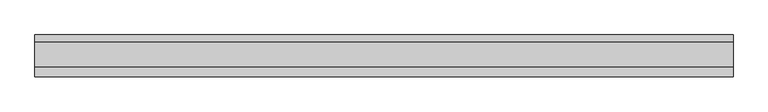
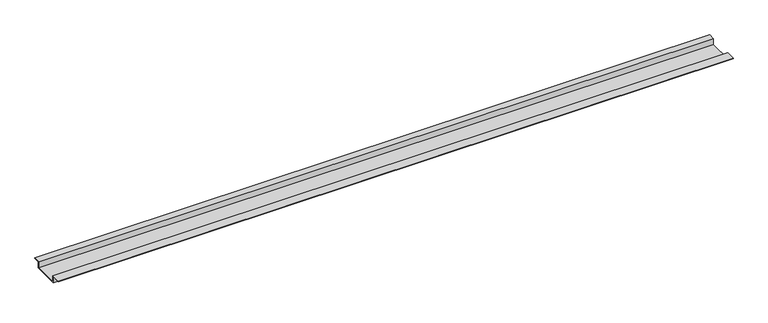
"""IFC4 building model written with IfcOpenShell, lengths in millimetres: proxy geometry, Soffit004 5682 : Soffit004 5682."""

from ifc_helpers import new_model, si_unit, frame, origin, place, context, project, spatial, polyline, outline, extrude, source, transform, mapped, element, save


def generic_models_106c7a7b(model_context):
    return source(origin(), model_context, "Body", "SweptSolid", [
        extrude(outline(polyline([(-5193.2078885, 39568.8162504), (-5193.2078885, 39549.7270423), (-5269.4066367, 39549.7270423), (-5269.4066367, 39568.8162502), (-5295.6622638, 39568.8162502), (-5295.6622638, 39570.0862502), (-5268.1366367, 39570.0862502), (-5268.1366367, 39550.996959), (-5194.4779718, 39550.996959), (-5194.4779718, 39570.0862504), (-5175.3485942, 39570.0862504), (-5175.3485942, 39568.8162504), (-5193.2078885, 39568.8162504)])), frame((12382.7678845, 0.0, 0.0), z_axis=(1.0, 0.0, 0.0), x_axis=(0.0, 1.0, 0.0)), (0.0, 0.0, 1.0), 2000.25),
    ])


if __name__ == "__main__":
    model = new_model("IFC4")
    model_context = context("Model", 3, world=origin())
    ifc_project = project(units=[si_unit("LENGTHUNIT", "METRE", prefix="MILLI")], contexts=[model_context])
    site = spatial("IfcSite", under=ifc_project)
    building = spatial("IfcBuilding", under=site)
    placement = place(None, origin())
    generic_models_shape = generic_models_106c7a7b(model_context)
    element("IfcBuildingElementProxy", 1, Name="Soffit004 5682 : Soffit004 5682", ObjectType="Soffit004 5682 : Soffit004 5682", at=placement, inside=building, context=model_context, shape_type="MappedRepresentation", body=[
        mapped(generic_models_shape, transform((0.0, 0.0, 0.0), x_axis=(1.0, 0.0, 0.0), y_axis=(0.0, 1.0, 0.0), z_axis=(0.0, 0.0, 1.0))),
    ])
    save(model, "model.ifc")

# Revit data of these elements
# Type "Soffit004 5682 : Soffit004 5682"
#   NameOverride = "Soffit004"
# Element 1 (IfcBuildingElementProxy, "Soffit004 5682 : Soffit004 5682")
#   Materials on its faces: "16 GA. COPPER SOFFIT VENT - VERIFY W/ ARCHITECT ON LOCATION"
# Materials
#   "16 GA. COPPER SOFFIT VENT - VERIFY W/ ARCHITECT ON LOCATION": class "Unassigned", colour RGB 85 255 127, transparency 0
